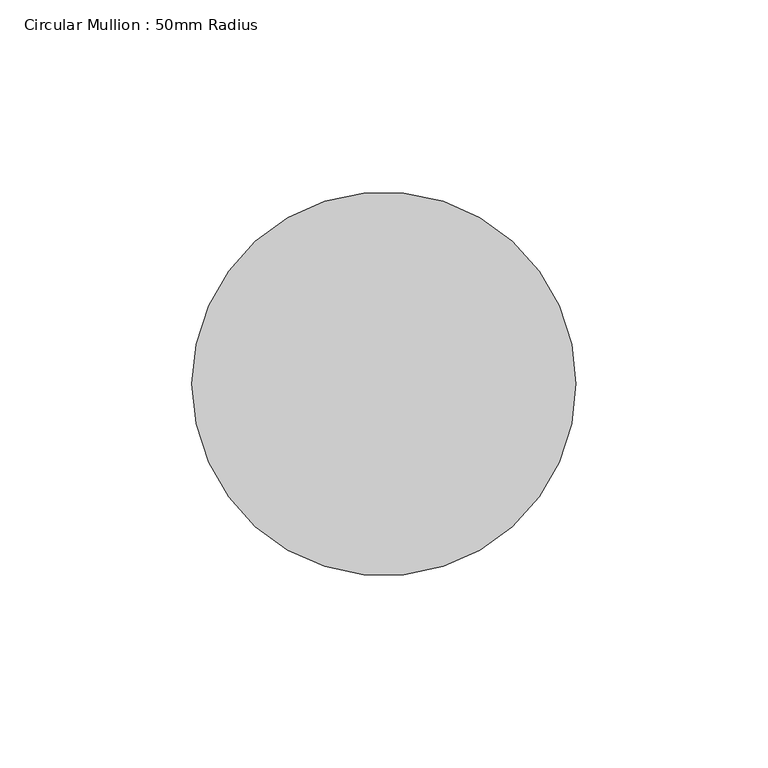
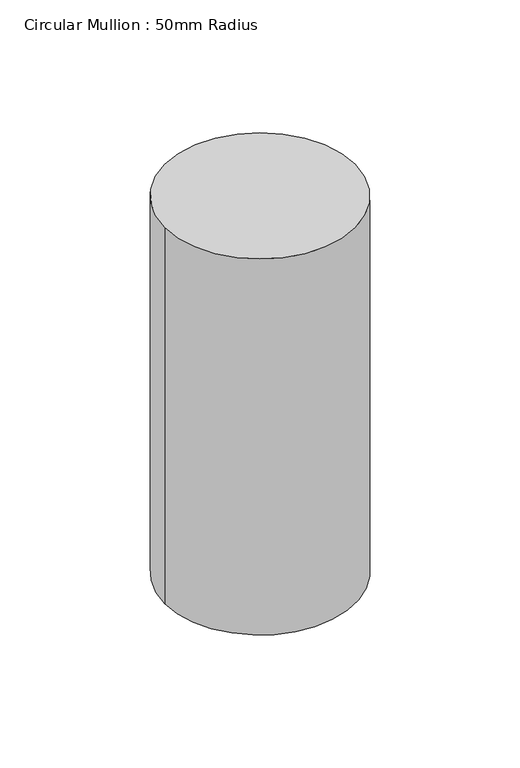
"""IFC4 building model written with IfcOpenShell, lengths in millimetres: member geometry, Circular Mullion : 50mm Radius."""

from ifc_helpers import new_model, si_unit, point, frame, origin, origin_2d, place, context, project, spatial, circle_curve, trimmed, segment, composite_curve, outline, extrude, source, transform, mapped, element, save


def circular_mullion_50mm_radius_6dbfb2e3(model_context):
    return source(origin(), model_context, "Body", "SweptSolid", [
        extrude(outline(composite_curve([segment(trimmed(circle_curve(origin_2d(), 50.0), [point((50.0, 0.0))], [point((-50.0, 0.0))], False, "CARTESIAN"), True, "CONTINUOUS"), segment(trimmed(circle_curve(origin_2d(), 50.0), [point((-50.0, 0.0))], [point((50.0, 0.0))], False, "CARTESIAN"), True, "CONTINUOUS")], self_intersect=False)), frame((0.0, 0.0, -208.906475), z_axis=(0.0, 0.0, 1.0), x_axis=(1.0, 0.0, 0.0)), (0.0, 0.0, 1.0), 208.906475),
    ])


if __name__ == "__main__":
    model = new_model("IFC4")
    model_context = context("Model", 3, world=origin())
    ifc_project = project(units=[si_unit("LENGTHUNIT", "METRE", prefix="MILLI")], contexts=[model_context])
    site = spatial("IfcSite", under=ifc_project)
    building = spatial("IfcBuilding", under=site)
    placement = place(None, origin())
    circular_mullion_50mm_radius_shape = circular_mullion_50mm_radius_6dbfb2e3(model_context)
    element("IfcMember", 1, ObjectType="Circular Mullion : 50mm Radius", at=placement, inside=building, context=model_context, shape_type="MappedRepresentation", body=[
        mapped(circular_mullion_50mm_radius_shape, transform((0.0, 0.0, 0.0), x_axis=(1.0, 0.0, 0.0), y_axis=(0.0, 1.0, 0.0), z_axis=(0.0, 0.0, 1.0))),
    ])
    save(model, "model.ifc")

# Revit data of these elements
# Type "Circular Mullion : 50mm Radius"
#   built-in parameter 1007350 = 0.164042 (stored number, unit not read)
# Element 1 (IfcMember, "Circular Mullion : 50mm Radius")
#   Materials on its faces: "Aluminium"
# Materials
#   "Aluminium": class "Metal", colour RGB 247 247 247, transparency 0, Description = "Aluminium 6061", Cost = 0
